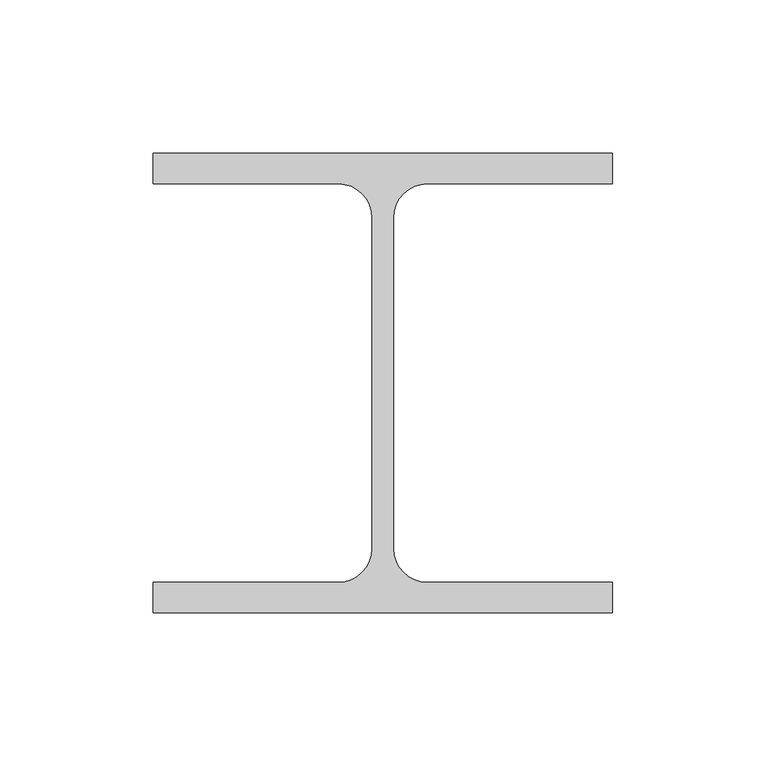
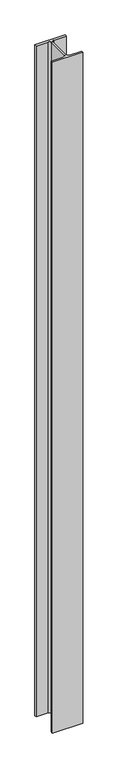
"""IFC4 building model written with IfcOpenShell, lengths in millimetres: column geometry, 0912_Steel Column_H_KSD3502 : H_SC_ASC_H-150x150x7x10."""

import ifcopenshell
import ifcopenshell.guid

model = None  # the IFC model being written
_history = None  # IfcOwnerHistory: only IFC2X3 demands one
_inside = {}  # id of a spatial element -> (the spatial element, [elements in it])
_under = {}  # id of a project, library or spatial element -> (it, [spatial elements below it])
_declared = {}  # id of a project -> (the project, [libraries it declares])
_typed = {}  # id of a type object -> (the type object, [elements of that type])
_made_of = {}  # id of a material, layer set ... -> (it, [elements and type objects made of it])


def new_model(schema):
    """Start an empty IFC model of exactly this schema.

    Asked for "IFC4X3", IfcOpenShell would pick the latest addendum, in which some entities
    have other attributes; the version numbers below select the first issue.
    IFC2X3 requires an IfcOwnerHistory on every rooted entity: one is made here for all.
    """
    global model, _history
    if schema == "IFC4X3":
        model = ifcopenshell.file(schema_version=(4, 3, 0, 0))
    else:
        model = ifcopenshell.file(schema=schema)
    _inside.clear()
    _under.clear()
    _declared.clear()
    _typed.clear()
    _made_of.clear()
    _history = None
    if model.schema == "IFC2X3":
        org = make("IfcOrganization", Name="unknown")
        user = make(
            "IfcPersonAndOrganization",
            ThePerson=make("IfcPerson", FamilyName="unknown"),
            TheOrganization=org,
        )
        app = make(
            "IfcApplication",
            ApplicationDeveloper=org,
            Version="unknown",
            ApplicationFullName="unknown",
            ApplicationIdentifier="unknown",
        )
        _history = make(
            "IfcOwnerHistory",
            OwningUser=user,
            OwningApplication=app,
            ChangeAction="ADDED",
            CreationDate=0,
        )
    return model


def make(cls, **values):
    """One entity of the class cls with the attributes given. An attribute that is None is left unset."""
    return model.create_entity(
        cls, **{name: value for name, value in values.items() if value is not None}
    )


def rooted(cls, **values):
    """An entity with a GlobalId (a new one), such as an element, a storey or a relation."""
    return make(cls, GlobalId=ifcopenshell.guid.new(), OwnerHistory=_history, **values)


def si_unit(unit_type, name, prefix=None):
    """IfcSIUnit, for example si_unit("LENGTHUNIT", "METRE", prefix="MILLI")."""
    return make("IfcSIUnit", UnitType=unit_type, Prefix=prefix, Name=name)


def assignment(units):
    """IfcUnitAssignment: the units of a project."""
    return None if units is None else make("IfcUnitAssignment", Units=units)


def point(xyz):
    """IfcCartesianPoint."""
    return None if xyz is None else make("IfcCartesianPoint", Coordinates=xyz)


def direction(xyz):
    """IfcDirection."""
    return None if xyz is None else make("IfcDirection", DirectionRatios=xyz)


def frame(location, z_axis=None, x_axis=None):
    """IfcAxis2Placement3D, a coordinate frame: its origin and axes. An axis left out is left unset."""
    return make(
        "IfcAxis2Placement3D",
        Location=point(location),
        Axis=direction(z_axis),
        RefDirection=direction(x_axis),
    )


def frame_2d(location, x_axis=None):
    """IfcAxis2Placement2D, a coordinate frame in the plane: its origin and x axis."""
    return make(
        "IfcAxis2Placement2D", Location=point(location), RefDirection=direction(x_axis)
    )


def origin():
    """The frame at (0, 0, 0) with its axes left unset."""
    return frame((0.0, 0.0, 0.0))


def place(relative_to, where):
    """IfcLocalPlacement: puts the frame where relative to a parent placement (None: the world)."""
    return make(
        "IfcLocalPlacement", PlacementRelTo=relative_to, RelativePlacement=where
    )


def context(
    kind, dimensions, precision=None, world=None, true_north=None, identifier=None
):
    """IfcGeometricRepresentationContext, for example the 3D "Model" context."""
    return make(
        "IfcGeometricRepresentationContext",
        ContextIdentifier=identifier,
        ContextType=kind,
        CoordinateSpaceDimension=dimensions,
        Precision=precision,
        WorldCoordinateSystem=world,
        TrueNorth=true_north,
    )


def project(units=None, contexts=None):
    """IfcProject with its units and contexts."""
    return rooted(
        "IfcProject",
        Name="project",
        RepresentationContexts=contexts,
        UnitsInContext=assignment(units),
    )


def spatial(cls, under=None, at=None, **own):
    """A site, building, storey or space (cls), placed at a placement, below another one or the project."""
    s = rooted(cls, ObjectPlacement=at, **own)
    if under is not None:
        _under.setdefault(under.id(), (under, []))[1].append(s)
    return s


def polyline(points):
    """IfcPolyline through the points."""
    return make("IfcPolyline", Points=[point(p) for p in points])


def circle_curve(where, radius):
    """IfcCircle in the frame where."""
    return make("IfcCircle", Position=where, Radius=radius)


def trimmed(basis, trim1, trim2, sense, master):
    """IfcTrimmedCurve: the piece of a basis curve between two trims."""
    return make(
        "IfcTrimmedCurve",
        BasisCurve=basis,
        Trim1=trim1,
        Trim2=trim2,
        SenseAgreement=sense,
        MasterRepresentation=master,
    )


def segment(curve, same_sense, transition):
    """IfcCompositeCurveSegment."""
    return make(
        "IfcCompositeCurveSegment",
        Transition=transition,
        SameSense=same_sense,
        ParentCurve=curve,
    )


def composite_curve(segments, self_intersect=None):
    """IfcCompositeCurve: segments joined end to end."""
    return make("IfcCompositeCurve", Segments=segments, SelfIntersect=self_intersect)


def outline(outer, holes=None, kind="AREA"):
    """IfcArbitraryClosedProfileDef: a profile drawn as a closed curve; with holes, ...WithVoids."""
    if holes is None:
        return make("IfcArbitraryClosedProfileDef", ProfileType=kind, OuterCurve=outer)
    return make(
        "IfcArbitraryProfileDefWithVoids",
        ProfileType=kind,
        OuterCurve=outer,
        InnerCurves=holes,
    )


def extrude(swept, where, along, depth):
    """IfcExtrudedAreaSolid: the profile swept, set in the frame where, extruded along a direction by depth."""
    return make(
        "IfcExtrudedAreaSolid",
        SweptArea=swept,
        Position=where,
        ExtrudedDirection=direction(along),
        Depth=depth,
    )


def shape(context_of_items, identifier, shape_type, items):
    """IfcShapeRepresentation: the items that make up one representation, for example the "Body"."""
    return make(
        "IfcShapeRepresentation",
        ContextOfItems=context_of_items,
        RepresentationIdentifier=identifier,
        RepresentationType=shape_type,
        Items=items,
    )


def source(mapping_origin, context_of_items, identifier, shape_type, items):
    """IfcRepresentationMap: a shape defined once, which mapped items show again and again."""
    return make(
        "IfcRepresentationMap",
        MappingOrigin=mapping_origin,
        MappedRepresentation=shape(context_of_items, identifier, shape_type, items),
    )


def transform(
    local_origin,
    x_axis=None,
    y_axis=None,
    z_axis=None,
    scale=None,
    scale2=None,
    scale3=None,
    uniform=True,
):
    """IfcCartesianTransformationOperator3D, or its non-uniform kind. x_axis, y_axis, z_axis: its Axis1, 2, 3."""
    if uniform:
        return make(
            "IfcCartesianTransformationOperator3D",
            Axis1=direction(x_axis),
            Axis2=direction(y_axis),
            LocalOrigin=point(local_origin),
            Scale=scale,
            Axis3=direction(z_axis),
        )
    return make(
        "IfcCartesianTransformationOperator3DnonUniform",
        Axis1=direction(x_axis),
        Axis2=direction(y_axis),
        LocalOrigin=point(local_origin),
        Scale=scale,
        Axis3=direction(z_axis),
        Scale2=scale2,
        Scale3=scale3,
    )


def mapped(mapping_source, mapping_target):
    """IfcMappedItem: shows the shape of a source again, moved by a transform."""
    return make(
        "IfcMappedItem", MappingSource=mapping_source, MappingTarget=mapping_target
    )


def made_of(thing, what):
    """Note that an element or type object is made of a material, layer set ...; save() writes the relation."""
    if what is not None:
        _made_of.setdefault(what.id(), (what, []))[1].append(thing)
    return thing


def element(
    cls,
    number,
    at=None,
    inside=None,
    cuts=None,
    type_object=None,
    material=None,
    context=None,
    identifier="Body",
    shape_type=None,
    held_by="IfcProductDefinitionShape",
    body=None,
    shapes=None,
    **own,
):
    """One element of the class cls, such as IfcWall. Its Tag is "e" and its number.

    at: its placement. inside: the storey or other place that contains it. cuts: it is an
    opening in that element (IfcRelVoidsElement). A single representation is given by context,
    identifier, shape_type and body (its items); several are given by shapes. held_by: the class
    of the entity that holds the representations. save() writes the other relations.
    """
    e = rooted(cls, Tag="e%d" % number, ObjectPlacement=at, **own)
    if body is not None:
        shapes = [shape(context, identifier, shape_type, body)]
    if shapes is not None:
        e.Representation = make(held_by, Representations=shapes)
    if inside is not None:
        _inside.setdefault(inside.id(), (inside, []))[1].append(e)
    if cuts is not None:
        rooted(
            "IfcRelVoidsElement", RelatingBuildingElement=cuts, RelatedOpeningElement=e
        )
    if type_object is not None:
        _typed.setdefault(type_object.id(), (type_object, []))[1].append(e)
    return made_of(e, material)


def aggregate(whole, parts):
    """IfcRelAggregates: a whole, such as a stair, and the parts it consists of."""
    return rooted("IfcRelAggregates", RelatingObject=whole, RelatedObjects=parts)


def save(model, path):
    """Write the relations noted so far, then the file.

    IfcRelAggregates (storeys below a building ...), IfcRelContainedInSpatialStructure (elements
    in a storey), IfcRelDefinesByType, IfcRelAssociatesMaterial and IfcRelDeclares: one each for
    every whole, place, type object, material and project.
    """
    for whole, parts in _under.values():
        aggregate(whole, parts)
    for where, things in _inside.values():
        rooted(
            "IfcRelContainedInSpatialStructure",
            RelatedElements=things,
            RelatingStructure=where,
        )
    for kind, things in _typed.values():
        rooted("IfcRelDefinesByType", RelatedObjects=things, RelatingType=kind)
    for what, things in _made_of.values():
        rooted("IfcRelAssociatesMaterial", RelatedObjects=things, RelatingMaterial=what)
    for by, libraries in _declared.values():
        rooted("IfcRelDeclares", RelatingContext=by, RelatedDefinitions=libraries)
    model.write(path)


def column_aafab9da(model_context):
    return source(origin(), model_context, "Body", "SweptSolid", [
        extrude(outline(composite_curve([segment(polyline([(75.0, 75.0), (75.0, 65.0), (14.5, 65.0)]), True, "CONTINUOUS"), segment(trimmed(circle_curve(frame_2d((14.5, 54.0)), 11.0), [point((14.5, 65.0))], [point((3.5, 54.0))], True, "CARTESIAN"), True, "CONTINUOUS"), segment(polyline([(3.5, 54.0), (3.5, -54.0)]), True, "CONTINUOUS"), segment(trimmed(circle_curve(frame_2d((14.5, -54.0)), 11.0), [point((3.5, -54.0))], [point((14.5, -65.0))], True, "CARTESIAN"), True, "CONTINUOUS"), segment(polyline([(14.5, -65.0), (75.0, -65.0), (75.0, -75.0), (-75.0, -75.0), (-75.0, -65.0), (-14.5, -65.0)]), True, "CONTINUOUS"), segment(trimmed(circle_curve(frame_2d((-14.5, -54.0)), 11.0), [point((-14.5, -65.0))], [point((-3.5, -54.0))], True, "CARTESIAN"), True, "CONTINUOUS"), segment(polyline([(-3.5, -54.0), (-3.5, 54.0)]), True, "CONTINUOUS"), segment(trimmed(circle_curve(frame_2d((-14.5, 54.0)), 11.0), [point((-3.5, 54.0))], [point((-14.5, 65.0))], True, "CARTESIAN"), True, "CONTINUOUS"), segment(polyline([(-14.5, 65.0), (-75.0, 65.0), (-75.0, 75.0), (75.0, 75.0)]), True, "CONTINUOUS")], self_intersect=False)), frame((0.0, 0.0, 4449.9720055), z_axis=(0.0, 0.0, 1.0), x_axis=(1.0, 0.0, 0.0)), (0.0, 0.0, 1.0), 3510.0),
    ])


if __name__ == "__main__":
    model = new_model("IFC4")
    model_context = context("Model", 3, world=origin())
    ifc_project = project(units=[si_unit("LENGTHUNIT", "METRE", prefix="MILLI")], contexts=[model_context])
    site = spatial("IfcSite", under=ifc_project)
    building = spatial("IfcBuilding", under=site)
    placement = place(None, origin())
    column_shape = column_aafab9da(model_context)
    element("IfcColumn", 1, ObjectType="0912_Steel Column_H_KSD3502 : H_SC_ASC_H-150x150x7x10", at=placement, inside=building, context=model_context, shape_type="MappedRepresentation", body=[
        mapped(column_shape, transform((0.0, 0.0, 0.0), x_axis=(1.0, 0.0, 0.0), y_axis=(0.0, 1.0, 0.0), z_axis=(0.0, 0.0, 1.0))),
    ])
    save(model, "model.ifc")

# Revit data of these elements
# Type "0912_Steel Column_H_KSD3502 : H_SC_ASC_H-150x150x7x10"
#   H_WM Code_1 = "S01AA002-00001 | Main Steel Structure Fabrication Work | Shelter/Building | Medium Steel - Standard (90KG/M>Weight≥30KG/M) | Material: (   )"
#   H_WM Code_2 = "S03AA028-00001 | Main Steel Structure Erection Work | Shelter/Building | Medium Steel (90KG/M>Weight≥30KG/M) | Material: (   )"
#   H_WM Code_3 = "S01AA010-00001 | Main Steel Structure Fabrication Work | Shelter/Building | Steel Painting/Coating | for Non-Fireproofed Steel Surface, Surface Preparation, Primer, Second & Final Coat | Material: (   )"
#   H_Q'ty Cal Type Tag = "SC-Q2"
#   Width = 15.0 cm
#   Web Thickness = 0.7 cm
#   Web Fillet = 1.1 cm
#   Warping Constant = 27562.5 cm⁶
#   Torsional Moment of Inertia = 11.6007 cm⁴
#   Section Area = 40.14 cm²
#   Plastic Modulus weak axis = 115.0 cm³
#   Plastic Modulus strong axis = 246.0 cm³
#   Perimeter = 0.87 m²/m
#   Nominal Weight = 31.50 kgf/m
#   Moment of Inertia weak axis = 563.00 cm⁴
#   Moment of Inertia strong axis = 1640.00 cm⁴
#   Height = 15.0 cm
#   Flange Thickness = 1.0 cm
#   Elastic Modulus weak axis = 75.1 cm³
#   Elastic Modulus strong axis = 219.0 cm³
#   Centroid Vertical = 7.5 cm
#   Centroid Horizontal = 7.5 cm
#   Structural Material [instance default] = Steel, 45-345
#   Section Name Key = ""
#   Bolt Spacing = 0
#   Assembly Code = ""
# Element 1 (IfcColumn, "0912_Steel Column_H_KSD3502 : H_SC_ASC_H-150x150x7x10")
#   Structural Material = none
# Materials
#   "Steel, 45-345": class "Metal", colour RGB 189 187 185, transparency 0, Description = "Steel 345 MPa", Cost = 0
